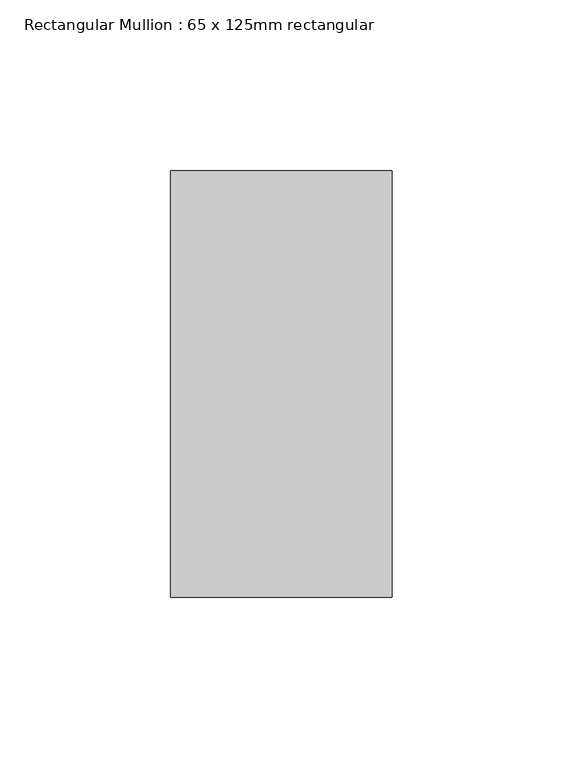
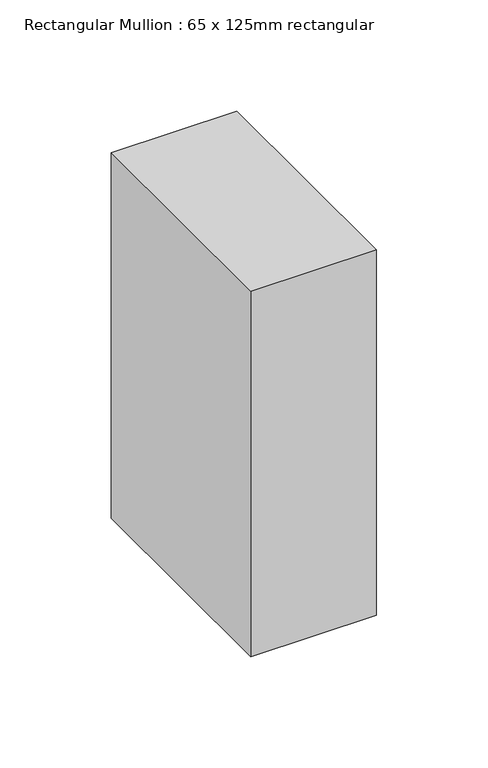
"""IFC4 building model written with IfcOpenShell, lengths in millimetres: member geometry, Rectangular Mullion : 65 x 125mm rectangular."""

from ifc_helpers import new_model, si_unit, frame, origin, place, context, project, spatial, polyline, outline, extrude, source, transform, mapped, element, save


def rectangular_mullion_65_x_125mm_rectangular_470365d3(model_context):
    return source(origin(), model_context, "Body", "SweptSolid", [
        extrude(outline(polyline([(32.5, 62.5), (32.5, -62.5), (-32.5, -62.5), (-32.5, 62.5), (32.5, 62.5)])), frame((0.0, 0.0, -200.0), z_axis=(0.0, 0.0, 1.0), x_axis=(1.0, 0.0, 0.0)), (0.0, 0.0, 1.0), 200.0),
    ])


if __name__ == "__main__":
    model = new_model("IFC4")
    model_context = context("Model", 3, world=origin())
    ifc_project = project(units=[si_unit("LENGTHUNIT", "METRE", prefix="MILLI")], contexts=[model_context])
    site = spatial("IfcSite", under=ifc_project)
    building = spatial("IfcBuilding", under=site)
    placement = place(None, origin())
    rectangular_mullion_65_x_125mm_rectangular_shape = rectangular_mullion_65_x_125mm_rectangular_470365d3(model_context)
    element("IfcMember", 1, ObjectType="Rectangular Mullion : 65 x 125mm rectangular", at=placement, inside=building, context=model_context, shape_type="MappedRepresentation", body=[
        mapped(rectangular_mullion_65_x_125mm_rectangular_shape, transform((0.0, 0.0, 0.0), x_axis=(1.0, 0.0, 0.0), y_axis=(0.0, 1.0, 0.0), z_axis=(0.0, 0.0, 1.0))),
    ])
    save(model, "model.ifc")

# Revit data of these elements
# Type "Rectangular Mullion : 65 x 125mm rectangular"
#   built-in parameter 1007304 = 0.410105 (stored number, unit not read)
#   built-in parameter 1007301 = 0.106627 (stored number, unit not read)
#   built-in parameter 1007300 = 0.106627 (stored number, unit not read)
# Element 1 (IfcMember, "Rectangular Mullion : 65 x 125mm rectangular")
#   Materials on its faces: "Aluminum"
# Materials
#   "Aluminum": class "Metal", colour RGB 244 245 246, transparency 0, Description = "Aluminum 6061", Cost = 0
